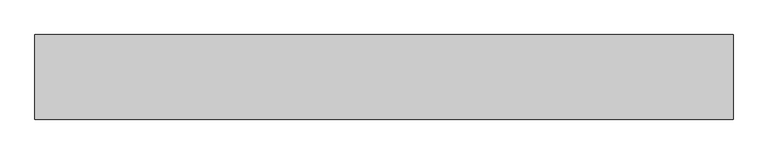
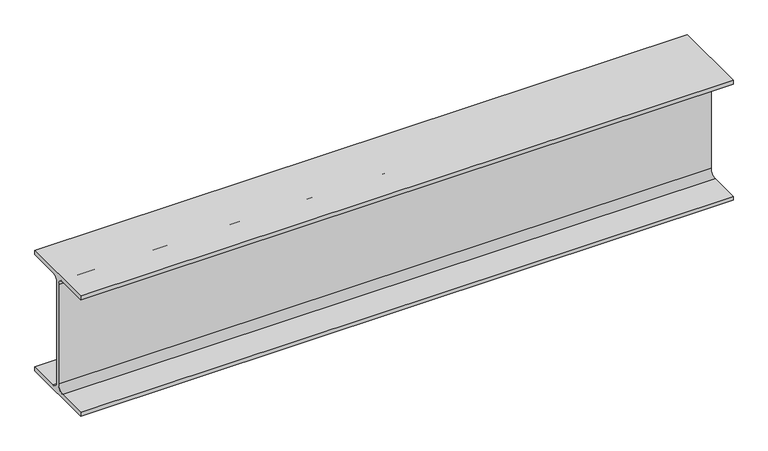
"""IFC4 building model written with IfcOpenShell, lengths in millimetres: beam geometry, 0912_Steel Framing_H-KSD3502 : H_SB_ASB_H-482x300x11x15."""

from ifc_helpers import new_model, si_unit, point, frame, frame_2d, origin, place, context, project, spatial, polyline, circle_curve, trimmed, segment, composite_curve, outline, extrude, source, transform, mapped, element, save


def beam_74d53594(model_context):
    return source(origin(), model_context, "Body", "SweptSolid", [
        extrude(outline(composite_curve([segment(polyline([(150.0, -226.0), (150.0, -241.0), (-150.0, -241.0), (-150.0, -226.0), (-31.5, -226.0)]), True, "CONTINUOUS"), segment(trimmed(circle_curve(frame_2d((-31.5, -200.0)), 26.0), [point((-31.5, -226.0))], [point((-5.5, -200.0))], True, "CARTESIAN"), True, "CONTINUOUS"), segment(polyline([(-5.5, -200.0), (-5.5, 200.0)]), True, "CONTINUOUS"), segment(trimmed(circle_curve(frame_2d((-31.5, 200.0)), 26.0), [point((-5.5, 200.0))], [point((-31.5, 226.0))], True, "CARTESIAN"), True, "CONTINUOUS"), segment(polyline([(-31.5, 226.0), (-150.0, 226.0), (-150.0, 241.0), (150.0, 241.0), (150.0, 226.0), (31.5, 226.0)]), True, "CONTINUOUS"), segment(trimmed(circle_curve(frame_2d((31.5, 200.0)), 26.0), [point((31.5, 226.0))], [point((5.5, 200.0))], True, "CARTESIAN"), True, "CONTINUOUS"), segment(polyline([(5.5, 200.0), (5.5, -200.0)]), True, "CONTINUOUS"), segment(trimmed(circle_curve(frame_2d((31.5, -200.0)), 26.0), [point((5.5, -200.0))], [point((31.5, -226.0))], True, "CARTESIAN"), True, "CONTINUOUS"), segment(polyline([(31.5, -226.0), (150.0, -226.0)]), True, "CONTINUOUS")], self_intersect=False)), frame((-1137.3, 0.0, 0.0), z_axis=(1.0, 0.0, 0.0), x_axis=(0.0, 1.0, 0.0)), (0.0, 0.0, 1.0), 2474.6),
    ])


if __name__ == "__main__":
    model = new_model("IFC4")
    model_context = context("Model", 3, world=origin())
    ifc_project = project(units=[si_unit("LENGTHUNIT", "METRE", prefix="MILLI")], contexts=[model_context])
    site = spatial("IfcSite", under=ifc_project)
    building = spatial("IfcBuilding", under=site)
    placement = place(None, origin())
    beam_shape = beam_74d53594(model_context)
    element("IfcBeam", 1, ObjectType="0912_Steel Framing_H-KSD3502 : H_SB_ASB_H-482x300x11x15", at=placement, inside=building, context=model_context, shape_type="MappedRepresentation", body=[
        mapped(beam_shape, transform((0.0, 0.0, 0.0), x_axis=(1.0, 0.0, 0.0), y_axis=(0.0, 1.0, 0.0), z_axis=(0.0, 0.0, 1.0))),
    ])
    save(model, "model.ifc")

# Revit data of these elements
# Type "0912_Steel Framing_H-KSD3502 : H_SB_ASB_H-482x300x11x15"
#   H_WM Code_1 = "S01AA001-00001 | Main Steel Structure Fabrication Work | Shelter/Building | Heavy Steel - Standard (Weight≥90KG/M) | Material: (   )"
#   H_WM Code_2 = "S03AA027-00001 | Main Steel Structure Erection Work | Shelter/Building | Heavy Steel (Weight≥90KG/M) | Material: (   )"
#   H_WM Code_3 = "S01AA010-00001 | Main Steel Structure Fabrication Work | Shelter/Building | Steel Painting/Coating | for Non-Fireproofed Steel Surface, Surface Preparation, Primer, Second & Final Coat | Material: (   )"
#   H_Q'ty Cal Type Tag = "SB-Q2"
#   Width = 30.0 cm
#   Web Thickness = 1.1 cm
#   Web Fillet = 2.6 cm
#   Warping Constant = 3680000.0 cm⁶
#   W = 0
#   Torsional Moment of Inertia = 88.2192 cm⁴
#   Section Area = 145.5 cm²
#   Plastic Modulus weak axis = 695.0 cm³
#   Plastic Modulus strong axis = 2790.0 cm³
#   Perimeter = 2.10 m²/m
#   Nominal Weight = 114.00 kgf/m
#   Moment of Inertia weak axis = 6760.00 cm⁴
#   Moment of Inertia strong axis = 60400.00 cm⁴
#   Height = 48.2 cm
#   Flange Thickness = 1.5 cm
#   Elastic Modulus weak axis = 451.0 cm³
#   Elastic Modulus strong axis = 2500.0 cm³
#   Centroid Vertical = 24.1 cm
#   Centroid Horizontal = 15.0 cm
#   Ix = 604000000
#   Length [instance default] = 1.5240 m
#   Zx = 2790000
#   b = 0.3000 m
#   h = 0.4820 m
#   r = 0.0260 m
#   s = 0.0110 m
#   t = 0.0150 m
#   A = 0.01455 m²
#   Structural Material [instance default] = Steel, 45-345
#   Assembly Code = ""
# Element 1 (IfcBeam, "0912_Steel Framing_H-KSD3502 : H_SB_ASB_H-482x300x11x15")
#   Structural Material = none
# Materials
#   "Steel, 45-345": class "Metal", colour RGB 189 187 185, transparency 0, Description = "Steel 345 MPa", Cost = 0
